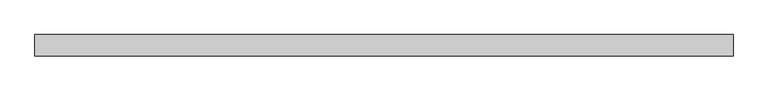
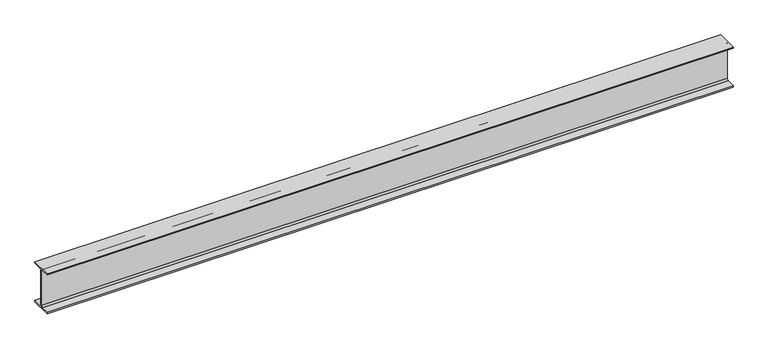
"""IFC4 building model written with IfcOpenShell, lengths in millimetres: beam geometry, 0912_Steel Framing_H-KSD3502 : H_SB_ASB_H-350x175x7x11."""

from ifc_helpers import new_model, si_unit, point, frame, frame_2d, origin, place, context, project, spatial, polyline, circle_curve, trimmed, segment, composite_curve, outline, extrude, source, transform, mapped, element, save


def beam_1864dd62(model_context):
    return source(origin(), model_context, "Body", "SweptSolid", [
        extrude(outline(composite_curve([segment(polyline([(87.5, -164.0), (87.5, -175.0), (-87.5, -175.0), (-87.5, -164.0), (-17.5, -164.0)]), True, "CONTINUOUS"), segment(trimmed(circle_curve(frame_2d((-17.5, -150.0)), 14.0), [point((-17.5, -164.0))], [point((-3.5, -150.0))], True, "CARTESIAN"), True, "CONTINUOUS"), segment(polyline([(-3.5, -150.0), (-3.5, 150.0)]), True, "CONTINUOUS"), segment(trimmed(circle_curve(frame_2d((-17.5, 150.0)), 14.0), [point((-3.5, 150.0))], [point((-17.5, 164.0))], True, "CARTESIAN"), True, "CONTINUOUS"), segment(polyline([(-17.5, 164.0), (-87.5, 164.0), (-87.5, 175.0), (87.5, 175.0), (87.5, 164.0), (17.5, 164.0)]), True, "CONTINUOUS"), segment(trimmed(circle_curve(frame_2d((17.5, 150.0)), 14.0), [point((17.5, 164.0))], [point((3.5, 150.0))], True, "CARTESIAN"), True, "CONTINUOUS"), segment(polyline([(3.5, 150.0), (3.5, -150.0)]), True, "CONTINUOUS"), segment(trimmed(circle_curve(frame_2d((17.5, -150.0)), 14.0), [point((3.5, -150.0))], [point((17.5, -164.0))], True, "CARTESIAN"), True, "CONTINUOUS"), segment(polyline([(17.5, -164.0), (87.5, -164.0)]), True, "CONTINUOUS")], self_intersect=False)), frame((-2837.3, 0.0, 0.0), z_axis=(1.0, 0.0, 0.0), x_axis=(0.0, 1.0, 0.0)), (0.0, 0.0, 1.0), 5674.6),
    ])


if __name__ == "__main__":
    model = new_model("IFC4")
    model_context = context("Model", 3, world=origin())
    ifc_project = project(units=[si_unit("LENGTHUNIT", "METRE", prefix="MILLI")], contexts=[model_context])
    site = spatial("IfcSite", under=ifc_project)
    building = spatial("IfcBuilding", under=site)
    placement = place(None, origin())
    beam_shape = beam_1864dd62(model_context)
    element("IfcBeam", 1, ObjectType="0912_Steel Framing_H-KSD3502 : H_SB_ASB_H-350x175x7x11", at=placement, inside=building, context=model_context, shape_type="MappedRepresentation", body=[
        mapped(beam_shape, transform((0.0, 0.0, 0.0), x_axis=(1.0, 0.0, 0.0), y_axis=(0.0, 1.0, 0.0), z_axis=(0.0, 0.0, 1.0))),
    ])
    save(model, "model.ifc")

# Revit data of these elements
# Type "0912_Steel Framing_H-KSD3502 : H_SB_ASB_H-350x175x7x11"
#   H_WM Code_1 = "S01AA002-00001 | Main Steel Structure Fabrication Work | Shelter/Building | Medium Steel - Standard (90KG/M>Weight≥30KG/M) | Material: (   )"
#   H_WM Code_2 = "S03AA028-00001 | Main Steel Structure Erection Work | Shelter/Building | Medium Steel (90KG/M>Weight≥30KG/M) | Material: (   )"
#   H_WM Code_3 = "S01AA010-00001 | Main Steel Structure Fabrication Work | Shelter/Building | Steel Painting/Coating | for Non-Fireproofed Steel Surface, Surface Preparation, Primer, Second & Final Coat | Material: (   )"
#   H_Q'ty Cal Type Tag = "SB-Q2"
#   Width = 17.5 cm
#   Web Thickness = 0.7 cm
#   Web Fillet = 1.4 cm
#   Warping Constant = 282000.0 cm⁶
#   W = 0
#   Torsional Moment of Inertia = 19.4042 cm⁴
#   Section Area = 63.14 cm²
#   Plastic Modulus weak axis = 174.0 cm³
#   Plastic Modulus strong axis = 868.0 cm³
#   Perimeter = 1.36 m²/m
#   Nominal Weight = 49.60 kgf/m
#   Moment of Inertia weak axis = 984.00 cm⁴
#   Moment of Inertia strong axis = 13600.00 cm⁴
#   Height = 35.0 cm
#   Flange Thickness = 1.1 cm
#   Elastic Modulus weak axis = 112.0 cm³
#   Elastic Modulus strong axis = 775.0 cm³
#   Centroid Vertical = 17.5 cm
#   Centroid Horizontal = 8.75 cm
#   Ix = 136000000
#   Length [instance default] = 1.5240 m
#   Zx = 868000
#   b = 0.1750 m
#   h = 0.3500 m
#   r = 0.0140 m
#   s = 0.0070 m
#   t = 0.0110 m
#   A = 0.006314 m²
#   Structural Material [instance default] = Steel, 45-345
#   Assembly Code = ""
# Element 1 (IfcBeam, "0912_Steel Framing_H-KSD3502 : H_SB_ASB_H-350x175x7x11")
#   Structural Material = none
# Materials
#   "Steel, 45-345": class "Metal", colour RGB 189 187 185, transparency 0, Description = "Steel 345 MPa", Cost = 0
